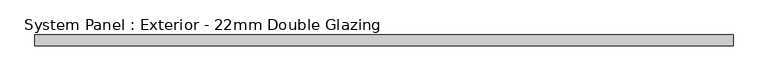
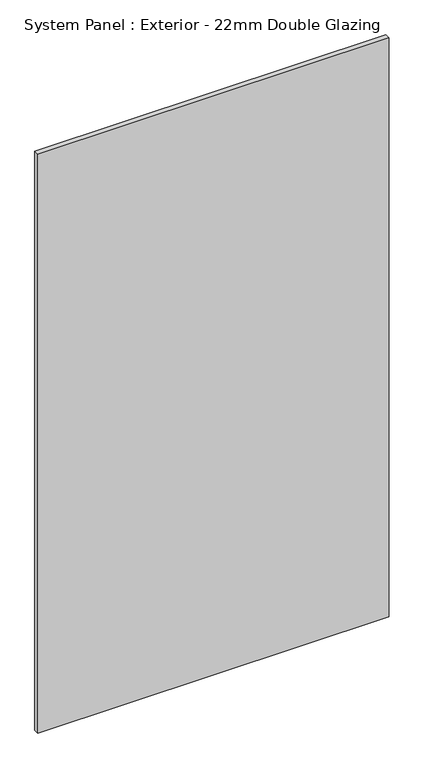
"""IFC4 building model written with IfcOpenShell, lengths in millimetres: plate geometry, System Panel : Exterior - 22mm Double Glazing."""

import ifcopenshell
import ifcopenshell.guid

model = None  # the IFC model being written
_history = None  # IfcOwnerHistory: only IFC2X3 demands one
_inside = {}  # id of a spatial element -> (the spatial element, [elements in it])
_under = {}  # id of a project, library or spatial element -> (it, [spatial elements below it])
_declared = {}  # id of a project -> (the project, [libraries it declares])
_typed = {}  # id of a type object -> (the type object, [elements of that type])
_made_of = {}  # id of a material, layer set ... -> (it, [elements and type objects made of it])


def new_model(schema):
    """Start an empty IFC model of exactly this schema.

    Asked for "IFC4X3", IfcOpenShell would pick the latest addendum, in which some entities
    have other attributes; the version numbers below select the first issue.
    IFC2X3 requires an IfcOwnerHistory on every rooted entity: one is made here for all.
    """
    global model, _history
    if schema == "IFC4X3":
        model = ifcopenshell.file(schema_version=(4, 3, 0, 0))
    else:
        model = ifcopenshell.file(schema=schema)
    _inside.clear()
    _under.clear()
    _declared.clear()
    _typed.clear()
    _made_of.clear()
    _history = None
    if model.schema == "IFC2X3":
        org = make("IfcOrganization", Name="unknown")
        user = make(
            "IfcPersonAndOrganization",
            ThePerson=make("IfcPerson", FamilyName="unknown"),
            TheOrganization=org,
        )
        app = make(
            "IfcApplication",
            ApplicationDeveloper=org,
            Version="unknown",
            ApplicationFullName="unknown",
            ApplicationIdentifier="unknown",
        )
        _history = make(
            "IfcOwnerHistory",
            OwningUser=user,
            OwningApplication=app,
            ChangeAction="ADDED",
            CreationDate=0,
        )
    return model


def make(cls, **values):
    """One entity of the class cls with the attributes given. An attribute that is None is left unset."""
    return model.create_entity(
        cls, **{name: value for name, value in values.items() if value is not None}
    )


def rooted(cls, **values):
    """An entity with a GlobalId (a new one), such as an element, a storey or a relation."""
    return make(cls, GlobalId=ifcopenshell.guid.new(), OwnerHistory=_history, **values)


def si_unit(unit_type, name, prefix=None):
    """IfcSIUnit, for example si_unit("LENGTHUNIT", "METRE", prefix="MILLI")."""
    return make("IfcSIUnit", UnitType=unit_type, Prefix=prefix, Name=name)


def assignment(units):
    """IfcUnitAssignment: the units of a project."""
    return None if units is None else make("IfcUnitAssignment", Units=units)


def point(xyz):
    """IfcCartesianPoint."""
    return None if xyz is None else make("IfcCartesianPoint", Coordinates=xyz)


def direction(xyz):
    """IfcDirection."""
    return None if xyz is None else make("IfcDirection", DirectionRatios=xyz)


def frame(location, z_axis=None, x_axis=None):
    """IfcAxis2Placement3D, a coordinate frame: its origin and axes. An axis left out is left unset."""
    return make(
        "IfcAxis2Placement3D",
        Location=point(location),
        Axis=direction(z_axis),
        RefDirection=direction(x_axis),
    )


def origin():
    """The frame at (0, 0, 0) with its axes left unset."""
    return frame((0.0, 0.0, 0.0))


def origin_with_axes():
    """The frame at (0, 0, 0) with the z axis (0, 0, 1) and the x axis (1, 0, 0) written out."""
    return frame((0.0, 0.0, 0.0), z_axis=(0.0, 0.0, 1.0), x_axis=(1.0, 0.0, 0.0))


def place(relative_to, where):
    """IfcLocalPlacement: puts the frame where relative to a parent placement (None: the world)."""
    return make(
        "IfcLocalPlacement", PlacementRelTo=relative_to, RelativePlacement=where
    )


def context(
    kind, dimensions, precision=None, world=None, true_north=None, identifier=None
):
    """IfcGeometricRepresentationContext, for example the 3D "Model" context."""
    return make(
        "IfcGeometricRepresentationContext",
        ContextIdentifier=identifier,
        ContextType=kind,
        CoordinateSpaceDimension=dimensions,
        Precision=precision,
        WorldCoordinateSystem=world,
        TrueNorth=true_north,
    )


def project(units=None, contexts=None):
    """IfcProject with its units and contexts."""
    return rooted(
        "IfcProject",
        Name="project",
        RepresentationContexts=contexts,
        UnitsInContext=assignment(units),
    )


def spatial(cls, under=None, at=None, **own):
    """A site, building, storey or space (cls), placed at a placement, below another one or the project."""
    s = rooted(cls, ObjectPlacement=at, **own)
    if under is not None:
        _under.setdefault(under.id(), (under, []))[1].append(s)
    return s


def polyline(points):
    """IfcPolyline through the points."""
    return make("IfcPolyline", Points=[point(p) for p in points])


def outline(outer, holes=None, kind="AREA"):
    """IfcArbitraryClosedProfileDef: a profile drawn as a closed curve; with holes, ...WithVoids."""
    if holes is None:
        return make("IfcArbitraryClosedProfileDef", ProfileType=kind, OuterCurve=outer)
    return make(
        "IfcArbitraryProfileDefWithVoids",
        ProfileType=kind,
        OuterCurve=outer,
        InnerCurves=holes,
    )


def extrude(swept, where, along, depth):
    """IfcExtrudedAreaSolid: the profile swept, set in the frame where, extruded along a direction by depth."""
    return make(
        "IfcExtrudedAreaSolid",
        SweptArea=swept,
        Position=where,
        ExtrudedDirection=direction(along),
        Depth=depth,
    )


def shape(context_of_items, identifier, shape_type, items):
    """IfcShapeRepresentation: the items that make up one representation, for example the "Body"."""
    return make(
        "IfcShapeRepresentation",
        ContextOfItems=context_of_items,
        RepresentationIdentifier=identifier,
        RepresentationType=shape_type,
        Items=items,
    )


def source(mapping_origin, context_of_items, identifier, shape_type, items):
    """IfcRepresentationMap: a shape defined once, which mapped items show again and again."""
    return make(
        "IfcRepresentationMap",
        MappingOrigin=mapping_origin,
        MappedRepresentation=shape(context_of_items, identifier, shape_type, items),
    )


def transform(
    local_origin,
    x_axis=None,
    y_axis=None,
    z_axis=None,
    scale=None,
    scale2=None,
    scale3=None,
    uniform=True,
):
    """IfcCartesianTransformationOperator3D, or its non-uniform kind. x_axis, y_axis, z_axis: its Axis1, 2, 3."""
    if uniform:
        return make(
            "IfcCartesianTransformationOperator3D",
            Axis1=direction(x_axis),
            Axis2=direction(y_axis),
            LocalOrigin=point(local_origin),
            Scale=scale,
            Axis3=direction(z_axis),
        )
    return make(
        "IfcCartesianTransformationOperator3DnonUniform",
        Axis1=direction(x_axis),
        Axis2=direction(y_axis),
        LocalOrigin=point(local_origin),
        Scale=scale,
        Axis3=direction(z_axis),
        Scale2=scale2,
        Scale3=scale3,
    )


def mapped(mapping_source, mapping_target):
    """IfcMappedItem: shows the shape of a source again, moved by a transform."""
    return make(
        "IfcMappedItem", MappingSource=mapping_source, MappingTarget=mapping_target
    )


def made_of(thing, what):
    """Note that an element or type object is made of a material, layer set ...; save() writes the relation."""
    if what is not None:
        _made_of.setdefault(what.id(), (what, []))[1].append(thing)
    return thing


def element(
    cls,
    number,
    at=None,
    inside=None,
    cuts=None,
    type_object=None,
    material=None,
    context=None,
    identifier="Body",
    shape_type=None,
    held_by="IfcProductDefinitionShape",
    body=None,
    shapes=None,
    **own,
):
    """One element of the class cls, such as IfcWall. Its Tag is "e" and its number.

    at: its placement. inside: the storey or other place that contains it. cuts: it is an
    opening in that element (IfcRelVoidsElement). A single representation is given by context,
    identifier, shape_type and body (its items); several are given by shapes. held_by: the class
    of the entity that holds the representations. save() writes the other relations.
    """
    e = rooted(cls, Tag="e%d" % number, ObjectPlacement=at, **own)
    if body is not None:
        shapes = [shape(context, identifier, shape_type, body)]
    if shapes is not None:
        e.Representation = make(held_by, Representations=shapes)
    if inside is not None:
        _inside.setdefault(inside.id(), (inside, []))[1].append(e)
    if cuts is not None:
        rooted(
            "IfcRelVoidsElement", RelatingBuildingElement=cuts, RelatedOpeningElement=e
        )
    if type_object is not None:
        _typed.setdefault(type_object.id(), (type_object, []))[1].append(e)
    return made_of(e, material)


def aggregate(whole, parts):
    """IfcRelAggregates: a whole, such as a stair, and the parts it consists of."""
    return rooted("IfcRelAggregates", RelatingObject=whole, RelatedObjects=parts)


def save(model, path):
    """Write the relations noted so far, then the file.

    IfcRelAggregates (storeys below a building ...), IfcRelContainedInSpatialStructure (elements
    in a storey), IfcRelDefinesByType, IfcRelAssociatesMaterial and IfcRelDeclares: one each for
    every whole, place, type object, material and project.
    """
    for whole, parts in _under.values():
        aggregate(whole, parts)
    for where, things in _inside.values():
        rooted(
            "IfcRelContainedInSpatialStructure",
            RelatedElements=things,
            RelatingStructure=where,
        )
    for kind, things in _typed.values():
        rooted("IfcRelDefinesByType", RelatedObjects=things, RelatingType=kind)
    for what, things in _made_of.values():
        rooted("IfcRelAssociatesMaterial", RelatedObjects=things, RelatingMaterial=what)
    for by, libraries in _declared.values():
        rooted("IfcRelDeclares", RelatingContext=by, RelatedDefinitions=libraries)
    model.write(path)


def system_panel_exterior_22mm_double_glazing_aa15faa2(model_context):
    return source(origin(), model_context, "Body", "SweptSolid", [
        extrude(outline(polyline([(724.9999999, 15.0), (-724.9999999, 15.0), (-724.9999999, 37.0), (724.9999999, 37.0), (724.9999999, 15.0)])), origin_with_axes(), (0.0, 0.0, 1.0), 2525.0),
    ])


if __name__ == "__main__":
    model = new_model("IFC4")
    model_context = context("Model", 3, world=origin())
    ifc_project = project(units=[si_unit("LENGTHUNIT", "METRE", prefix="MILLI")], contexts=[model_context])
    site = spatial("IfcSite", under=ifc_project)
    building = spatial("IfcBuilding", under=site)
    placement = place(None, origin())
    system_panel_exterior_22mm_double_glazing_shape = system_panel_exterior_22mm_double_glazing_aa15faa2(model_context)
    element("IfcPlate", 1, ObjectType="System Panel : Exterior - 22mm Double Glazing", at=placement, inside=building, context=model_context, shape_type="MappedRepresentation", body=[
        mapped(system_panel_exterior_22mm_double_glazing_shape, transform((0.0, 0.0, 0.0), x_axis=(1.0, 0.0, 0.0), y_axis=(0.0, 1.0, 0.0), z_axis=(0.0, 0.0, 1.0))),
    ])
    save(model, "model.ifc")

# Revit data of these elements
# Element 1 (IfcPlate, "System Panel : Exterior - 22mm Double Glazing")
#   Materials on its faces: "Glass"
# Materials
#   "Glass": class "Glass", colour RGB 180 200 255, transparency 0.75, Description = "Generisk glas", Cost = 0
